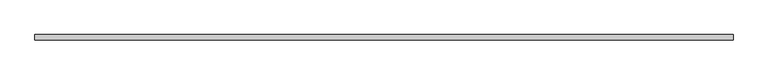
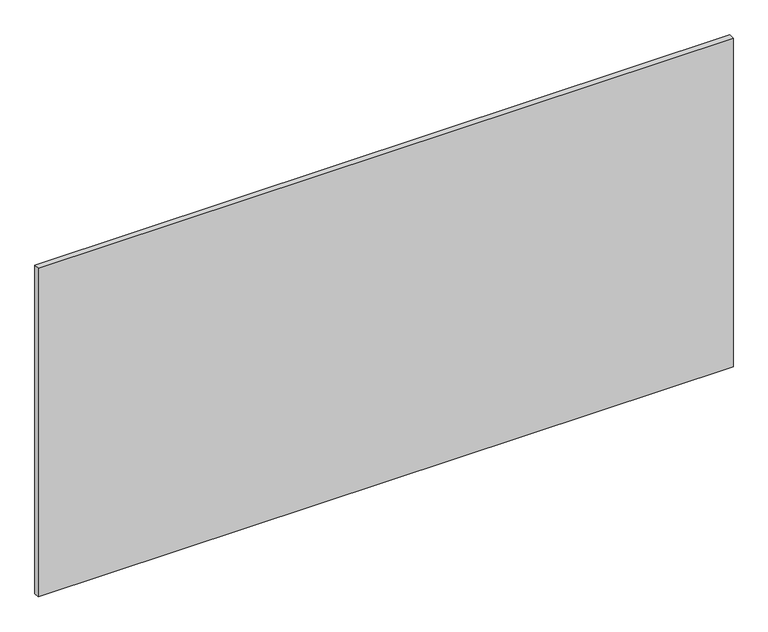
"""IFC4 building model written with IfcOpenShell, lengths in millimetres: proxy geometry, Inner panel:Inner panel:1:Inner panel:1 : Inner panel:Inner panel:300324:300043:Inner panel:1:Inner panel:1 : Inner panel:Inner panel:300324:300043 : Inner panel:Inner panel:1:Inner panel:1 : Inner panel:Inner panel:300324:300043:23 : Inner panel:Inner panel:1:Inner panel:1 : Inner panel:Inner panel:300324:300043:Inner panel:1:Inner panel:1 : Inner panel:Inner panel:300324:300043 : Inner panel:Inner panel:1:Inner panel:1 : Inner panel:Inner panel:300324:300043:300031."""

import ifcopenshell
import ifcopenshell.guid

model = None  # the IFC model being written
_history = None  # IfcOwnerHistory: only IFC2X3 demands one
_inside = {}  # id of a spatial element -> (the spatial element, [elements in it])
_under = {}  # id of a project, library or spatial element -> (it, [spatial elements below it])
_declared = {}  # id of a project -> (the project, [libraries it declares])
_typed = {}  # id of a type object -> (the type object, [elements of that type])
_made_of = {}  # id of a material, layer set ... -> (it, [elements and type objects made of it])


def new_model(schema):
    """Start an empty IFC model of exactly this schema.

    Asked for "IFC4X3", IfcOpenShell would pick the latest addendum, in which some entities
    have other attributes; the version numbers below select the first issue.
    IFC2X3 requires an IfcOwnerHistory on every rooted entity: one is made here for all.
    """
    global model, _history
    if schema == "IFC4X3":
        model = ifcopenshell.file(schema_version=(4, 3, 0, 0))
    else:
        model = ifcopenshell.file(schema=schema)
    _inside.clear()
    _under.clear()
    _declared.clear()
    _typed.clear()
    _made_of.clear()
    _history = None
    if model.schema == "IFC2X3":
        org = make("IfcOrganization", Name="unknown")
        user = make(
            "IfcPersonAndOrganization",
            ThePerson=make("IfcPerson", FamilyName="unknown"),
            TheOrganization=org,
        )
        app = make(
            "IfcApplication",
            ApplicationDeveloper=org,
            Version="unknown",
            ApplicationFullName="unknown",
            ApplicationIdentifier="unknown",
        )
        _history = make(
            "IfcOwnerHistory",
            OwningUser=user,
            OwningApplication=app,
            ChangeAction="ADDED",
            CreationDate=0,
        )
    return model


def make(cls, **values):
    """One entity of the class cls with the attributes given. An attribute that is None is left unset."""
    return model.create_entity(
        cls, **{name: value for name, value in values.items() if value is not None}
    )


def rooted(cls, **values):
    """An entity with a GlobalId (a new one), such as an element, a storey or a relation."""
    return make(cls, GlobalId=ifcopenshell.guid.new(), OwnerHistory=_history, **values)


def si_unit(unit_type, name, prefix=None):
    """IfcSIUnit, for example si_unit("LENGTHUNIT", "METRE", prefix="MILLI")."""
    return make("IfcSIUnit", UnitType=unit_type, Prefix=prefix, Name=name)


def assignment(units):
    """IfcUnitAssignment: the units of a project."""
    return None if units is None else make("IfcUnitAssignment", Units=units)


def point(xyz):
    """IfcCartesianPoint."""
    return None if xyz is None else make("IfcCartesianPoint", Coordinates=xyz)


def direction(xyz):
    """IfcDirection."""
    return None if xyz is None else make("IfcDirection", DirectionRatios=xyz)


def frame(location, z_axis=None, x_axis=None):
    """IfcAxis2Placement3D, a coordinate frame: its origin and axes. An axis left out is left unset."""
    return make(
        "IfcAxis2Placement3D",
        Location=point(location),
        Axis=direction(z_axis),
        RefDirection=direction(x_axis),
    )


def origin():
    """The frame at (0, 0, 0) with its axes left unset."""
    return frame((0.0, 0.0, 0.0))


def place(relative_to, where):
    """IfcLocalPlacement: puts the frame where relative to a parent placement (None: the world)."""
    return make(
        "IfcLocalPlacement", PlacementRelTo=relative_to, RelativePlacement=where
    )


def context(
    kind, dimensions, precision=None, world=None, true_north=None, identifier=None
):
    """IfcGeometricRepresentationContext, for example the 3D "Model" context."""
    return make(
        "IfcGeometricRepresentationContext",
        ContextIdentifier=identifier,
        ContextType=kind,
        CoordinateSpaceDimension=dimensions,
        Precision=precision,
        WorldCoordinateSystem=world,
        TrueNorth=true_north,
    )


def project(units=None, contexts=None):
    """IfcProject with its units and contexts."""
    return rooted(
        "IfcProject",
        Name="project",
        RepresentationContexts=contexts,
        UnitsInContext=assignment(units),
    )


def spatial(cls, under=None, at=None, **own):
    """A site, building, storey or space (cls), placed at a placement, below another one or the project."""
    s = rooted(cls, ObjectPlacement=at, **own)
    if under is not None:
        _under.setdefault(under.id(), (under, []))[1].append(s)
    return s


def polyline(points):
    """IfcPolyline through the points."""
    return make("IfcPolyline", Points=[point(p) for p in points])


def outline(outer, holes=None, kind="AREA"):
    """IfcArbitraryClosedProfileDef: a profile drawn as a closed curve; with holes, ...WithVoids."""
    if holes is None:
        return make("IfcArbitraryClosedProfileDef", ProfileType=kind, OuterCurve=outer)
    return make(
        "IfcArbitraryProfileDefWithVoids",
        ProfileType=kind,
        OuterCurve=outer,
        InnerCurves=holes,
    )


def extrude(swept, where, along, depth):
    """IfcExtrudedAreaSolid: the profile swept, set in the frame where, extruded along a direction by depth."""
    return make(
        "IfcExtrudedAreaSolid",
        SweptArea=swept,
        Position=where,
        ExtrudedDirection=direction(along),
        Depth=depth,
    )


def shape(context_of_items, identifier, shape_type, items):
    """IfcShapeRepresentation: the items that make up one representation, for example the "Body"."""
    return make(
        "IfcShapeRepresentation",
        ContextOfItems=context_of_items,
        RepresentationIdentifier=identifier,
        RepresentationType=shape_type,
        Items=items,
    )


def source(mapping_origin, context_of_items, identifier, shape_type, items):
    """IfcRepresentationMap: a shape defined once, which mapped items show again and again."""
    return make(
        "IfcRepresentationMap",
        MappingOrigin=mapping_origin,
        MappedRepresentation=shape(context_of_items, identifier, shape_type, items),
    )


def transform(
    local_origin,
    x_axis=None,
    y_axis=None,
    z_axis=None,
    scale=None,
    scale2=None,
    scale3=None,
    uniform=True,
):
    """IfcCartesianTransformationOperator3D, or its non-uniform kind. x_axis, y_axis, z_axis: its Axis1, 2, 3."""
    if uniform:
        return make(
            "IfcCartesianTransformationOperator3D",
            Axis1=direction(x_axis),
            Axis2=direction(y_axis),
            LocalOrigin=point(local_origin),
            Scale=scale,
            Axis3=direction(z_axis),
        )
    return make(
        "IfcCartesianTransformationOperator3DnonUniform",
        Axis1=direction(x_axis),
        Axis2=direction(y_axis),
        LocalOrigin=point(local_origin),
        Scale=scale,
        Axis3=direction(z_axis),
        Scale2=scale2,
        Scale3=scale3,
    )


def mapped(mapping_source, mapping_target):
    """IfcMappedItem: shows the shape of a source again, moved by a transform."""
    return make(
        "IfcMappedItem", MappingSource=mapping_source, MappingTarget=mapping_target
    )


def made_of(thing, what):
    """Note that an element or type object is made of a material, layer set ...; save() writes the relation."""
    if what is not None:
        _made_of.setdefault(what.id(), (what, []))[1].append(thing)
    return thing


def element(
    cls,
    number,
    at=None,
    inside=None,
    cuts=None,
    type_object=None,
    material=None,
    context=None,
    identifier="Body",
    shape_type=None,
    held_by="IfcProductDefinitionShape",
    body=None,
    shapes=None,
    **own,
):
    """One element of the class cls, such as IfcWall. Its Tag is "e" and its number.

    at: its placement. inside: the storey or other place that contains it. cuts: it is an
    opening in that element (IfcRelVoidsElement). A single representation is given by context,
    identifier, shape_type and body (its items); several are given by shapes. held_by: the class
    of the entity that holds the representations. save() writes the other relations.
    """
    e = rooted(cls, Tag="e%d" % number, ObjectPlacement=at, **own)
    if body is not None:
        shapes = [shape(context, identifier, shape_type, body)]
    if shapes is not None:
        e.Representation = make(held_by, Representations=shapes)
    if inside is not None:
        _inside.setdefault(inside.id(), (inside, []))[1].append(e)
    if cuts is not None:
        rooted(
            "IfcRelVoidsElement", RelatingBuildingElement=cuts, RelatedOpeningElement=e
        )
    if type_object is not None:
        _typed.setdefault(type_object.id(), (type_object, []))[1].append(e)
    return made_of(e, material)


def aggregate(whole, parts):
    """IfcRelAggregates: a whole, such as a stair, and the parts it consists of."""
    return rooted("IfcRelAggregates", RelatingObject=whole, RelatedObjects=parts)


def save(model, path):
    """Write the relations noted so far, then the file.

    IfcRelAggregates (storeys below a building ...), IfcRelContainedInSpatialStructure (elements
    in a storey), IfcRelDefinesByType, IfcRelAssociatesMaterial and IfcRelDeclares: one each for
    every whole, place, type object, material and project.
    """
    for whole, parts in _under.values():
        aggregate(whole, parts)
    for where, things in _inside.values():
        rooted(
            "IfcRelContainedInSpatialStructure",
            RelatedElements=things,
            RelatingStructure=where,
        )
    for kind, things in _typed.values():
        rooted("IfcRelDefinesByType", RelatedObjects=things, RelatingType=kind)
    for what, things in _made_of.values():
        rooted("IfcRelAssociatesMaterial", RelatedObjects=things, RelatingMaterial=what)
    for by, libraries in _declared.values():
        rooted("IfcRelDeclares", RelatingContext=by, RelatedDefinitions=libraries)
    model.write(path)


def generic_models_f2ad3a79(model_context):
    return source(origin(), model_context, "Body", "SweptSolid", [
        extrude(outline(polyline([(591293.3367236, -567913.5913841), (593731.7367236, -567913.5913841), (593731.7367236, -567932.6413841), (591293.3367236, -567932.6413841), (591293.3367236, -567913.5913841)])), frame((0.0, 0.0, 2495.55), z_axis=(0.0, 0.0, 1.0), x_axis=(1.0, 0.0, 0.0)), (0.0, 0.0, 1.0), 1219.2),
    ])


if __name__ == "__main__":
    model = new_model("IFC4")
    model_context = context("Model", 3, world=origin())
    ifc_project = project(units=[si_unit("LENGTHUNIT", "METRE", prefix="MILLI")], contexts=[model_context])
    site = spatial("IfcSite", under=ifc_project)
    building = spatial("IfcBuilding", under=site)
    placement = place(None, origin())
    generic_models_shape = generic_models_f2ad3a79(model_context)
    element("IfcBuildingElementProxy", 1, Name="Inner panel:Inner panel:1:Inner panel:1 : Inner panel:Inner panel:300324:300043:Inner panel:1:Inner panel:1 : Inner panel:Inner panel:300324:300043 : Inner panel:Inner panel:1:Inner panel:1 : Inner panel:Inner panel:300324:300043:23 : Inner panel:Inner panel:1:Inner panel:1 : Inner panel:Inner panel:300324:300043:Inner panel:1:Inner panel:1 : Inner panel:Inner panel:300324:300043 : Inner panel:Inner panel:1:Inner panel:1 : Inner panel:Inner panel:300324:300043:300031", ObjectType="Inner panel:Inner panel:1:Inner panel:1 : Inner panel:Inner panel:300324:300043:Inner panel:1:Inner panel:1 : Inner panel:Inner panel:300324:300043 : Inner panel:Inner panel:1:Inner panel:1 : Inner panel:Inner panel:300324:300043:23 : Inner panel:Inner panel:1:Inner panel:1 : Inner panel:Inner panel:300324:300043:Inner panel:1:Inner panel:1 : Inner panel:Inner panel:300324:300043 : Inner panel:Inner panel:1:Inner panel:1 : Inner panel:Inner panel:300324:300043:300031", at=placement, inside=building, context=model_context, shape_type="MappedRepresentation", body=[
        mapped(generic_models_shape, transform((0.0, 0.0, 0.0), x_axis=(1.0, 0.0, 0.0), y_axis=(0.0, 1.0, 0.0), z_axis=(0.0, 0.0, 1.0))),
    ])
    save(model, "model.ifc")

# Revit data of these elements
# Type "Inner panel:Inner panel:1:Inner panel:1 : Inner panel:Inner panel:300324:300043:Inner panel:1:Inner panel:1 : Inner panel:Inner panel:300324:300043 : Inner panel:Inner panel:1:Inner panel:1 : Inner panel:Inner panel:300324:300043:23 : Inner panel:Inner panel:1:Inner panel:1 : Inner panel:Inner panel:300324:300043:Inner panel:1:Inner panel:1 : Inner panel:Inner panel:300324:300043 : Inner panel:Inner panel:1:Inner panel:1 : Inner panel:Inner panel:300324:300043:300031"
#   NameOverride = "Inner panel:Inner panel:1:Inner panel:1 : Inner panel:Inner panel:300324:300043:Inner panel:1:Inner panel:1 : Inner panel:Inner panel:300324:300043 : Inner panel:Inner panel:1:Inner panel:1 : Inner panel:Inner panel:300324:300043:300031"
#   ObjectTypeOverride = "Inner panel:1:Inner panel:1 : Inner panel:Inner panel:300324:300043 : Inner panel:Inner panel:1:Inner panel:1 : Inner panel:Inner panel:300324:300043"
#   Reference = "Inner panel"
#   Tag = "300031"
# Element 1 (IfcBuildingElementProxy, "Inner panel:Inner panel:1:Inner panel:1 : Inner panel:Inner panel:300324:300043:Inner panel:1:Inner panel:1 : Inner panel:Inner panel:300324:300043 : Inner panel:Inner panel:1:Inner panel:1 : Inner panel:Inner panel:300324:300043:23 : Inner panel:Inner panel:1:Inner panel:1 : Inner panel:Inner panel:300324:300043:Inner panel:1:Inner panel:1 : Inner panel:Inner panel:300324:300043 : Inner panel:Inner panel:1:Inner panel:1 : Inner panel:Inner panel:300324:300043:300031")
#   Materials on its faces: "3/4\" PREFINISHED STAINED/SEALED PLYWOOD (FINISH: GRADE B,  FLAME SPREAD: CLASS B)"
# Materials
#   "3/4\" PREFINISHED STAINED/SEALED PLYWOOD (FINISH: GRADE B,  FLAME SPREAD: CLASS B)": class "Wood", colour RGB 149 120 74, transparency 0, Description = "Plywood, sheathing grade", Cost = 0
